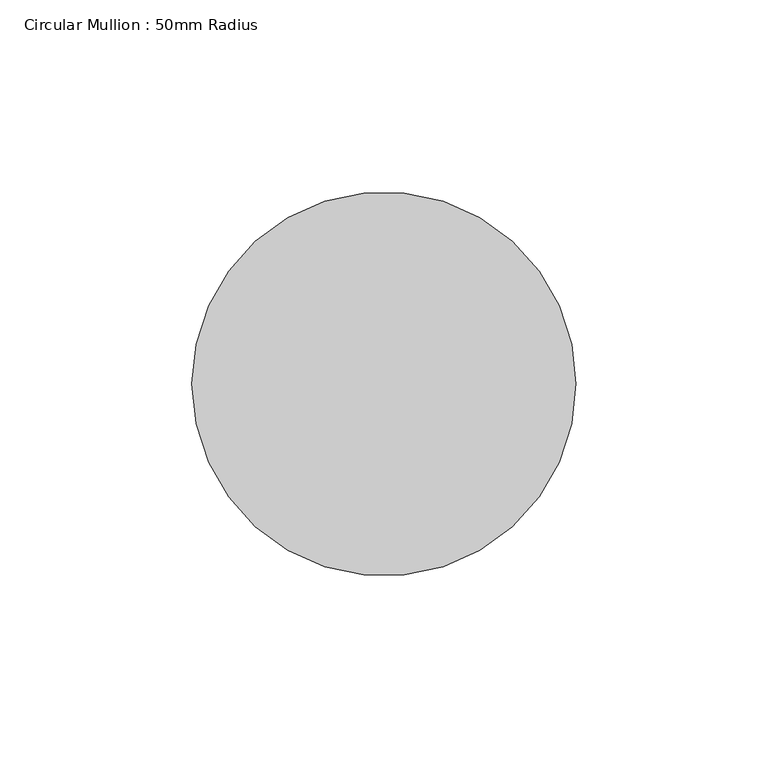
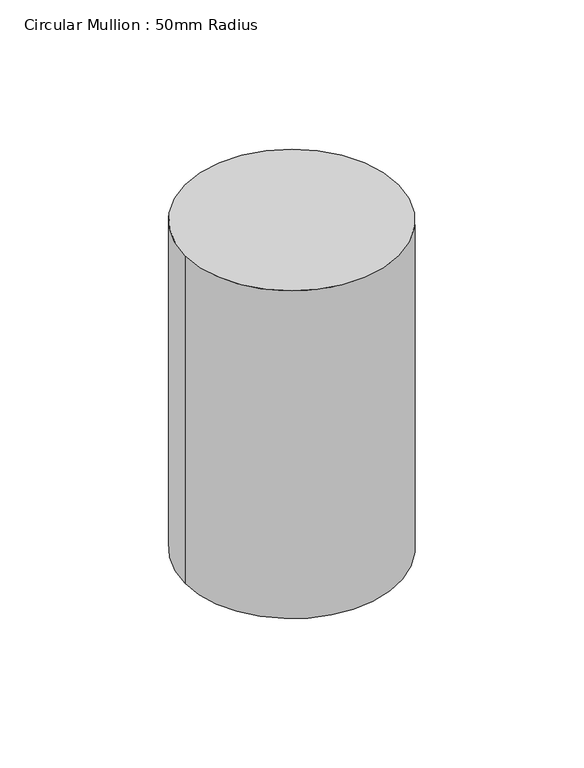
"""IFC4 building model written with IfcOpenShell, lengths in millimetres: member geometry, Circular Mullion : 50mm Radius."""

import ifcopenshell
import ifcopenshell.guid

model = None  # the IFC model being written
_history = None  # IfcOwnerHistory: only IFC2X3 demands one
_inside = {}  # id of a spatial element -> (the spatial element, [elements in it])
_under = {}  # id of a project, library or spatial element -> (it, [spatial elements below it])
_declared = {}  # id of a project -> (the project, [libraries it declares])
_typed = {}  # id of a type object -> (the type object, [elements of that type])
_made_of = {}  # id of a material, layer set ... -> (it, [elements and type objects made of it])


def new_model(schema):
    """Start an empty IFC model of exactly this schema.

    Asked for "IFC4X3", IfcOpenShell would pick the latest addendum, in which some entities
    have other attributes; the version numbers below select the first issue.
    IFC2X3 requires an IfcOwnerHistory on every rooted entity: one is made here for all.
    """
    global model, _history
    if schema == "IFC4X3":
        model = ifcopenshell.file(schema_version=(4, 3, 0, 0))
    else:
        model = ifcopenshell.file(schema=schema)
    _inside.clear()
    _under.clear()
    _declared.clear()
    _typed.clear()
    _made_of.clear()
    _history = None
    if model.schema == "IFC2X3":
        org = make("IfcOrganization", Name="unknown")
        user = make(
            "IfcPersonAndOrganization",
            ThePerson=make("IfcPerson", FamilyName="unknown"),
            TheOrganization=org,
        )
        app = make(
            "IfcApplication",
            ApplicationDeveloper=org,
            Version="unknown",
            ApplicationFullName="unknown",
            ApplicationIdentifier="unknown",
        )
        _history = make(
            "IfcOwnerHistory",
            OwningUser=user,
            OwningApplication=app,
            ChangeAction="ADDED",
            CreationDate=0,
        )
    return model


def make(cls, **values):
    """One entity of the class cls with the attributes given. An attribute that is None is left unset."""
    return model.create_entity(
        cls, **{name: value for name, value in values.items() if value is not None}
    )


def rooted(cls, **values):
    """An entity with a GlobalId (a new one), such as an element, a storey or a relation."""
    return make(cls, GlobalId=ifcopenshell.guid.new(), OwnerHistory=_history, **values)


def si_unit(unit_type, name, prefix=None):
    """IfcSIUnit, for example si_unit("LENGTHUNIT", "METRE", prefix="MILLI")."""
    return make("IfcSIUnit", UnitType=unit_type, Prefix=prefix, Name=name)


def assignment(units):
    """IfcUnitAssignment: the units of a project."""
    return None if units is None else make("IfcUnitAssignment", Units=units)


def point(xyz):
    """IfcCartesianPoint."""
    return None if xyz is None else make("IfcCartesianPoint", Coordinates=xyz)


def direction(xyz):
    """IfcDirection."""
    return None if xyz is None else make("IfcDirection", DirectionRatios=xyz)


def frame(location, z_axis=None, x_axis=None):
    """IfcAxis2Placement3D, a coordinate frame: its origin and axes. An axis left out is left unset."""
    return make(
        "IfcAxis2Placement3D",
        Location=point(location),
        Axis=direction(z_axis),
        RefDirection=direction(x_axis),
    )


def frame_2d(location, x_axis=None):
    """IfcAxis2Placement2D, a coordinate frame in the plane: its origin and x axis."""
    return make(
        "IfcAxis2Placement2D", Location=point(location), RefDirection=direction(x_axis)
    )


def origin():
    """The frame at (0, 0, 0) with its axes left unset."""
    return frame((0.0, 0.0, 0.0))


def origin_2d():
    """The frame at (0, 0) in the plane with its x axis left unset."""
    return frame_2d((0.0, 0.0))


def place(relative_to, where):
    """IfcLocalPlacement: puts the frame where relative to a parent placement (None: the world)."""
    return make(
        "IfcLocalPlacement", PlacementRelTo=relative_to, RelativePlacement=where
    )


def context(
    kind, dimensions, precision=None, world=None, true_north=None, identifier=None
):
    """IfcGeometricRepresentationContext, for example the 3D "Model" context."""
    return make(
        "IfcGeometricRepresentationContext",
        ContextIdentifier=identifier,
        ContextType=kind,
        CoordinateSpaceDimension=dimensions,
        Precision=precision,
        WorldCoordinateSystem=world,
        TrueNorth=true_north,
    )


def project(units=None, contexts=None):
    """IfcProject with its units and contexts."""
    return rooted(
        "IfcProject",
        Name="project",
        RepresentationContexts=contexts,
        UnitsInContext=assignment(units),
    )


def spatial(cls, under=None, at=None, **own):
    """A site, building, storey or space (cls), placed at a placement, below another one or the project."""
    s = rooted(cls, ObjectPlacement=at, **own)
    if under is not None:
        _under.setdefault(under.id(), (under, []))[1].append(s)
    return s


def circle_curve(where, radius):
    """IfcCircle in the frame where."""
    return make("IfcCircle", Position=where, Radius=radius)


def trimmed(basis, trim1, trim2, sense, master):
    """IfcTrimmedCurve: the piece of a basis curve between two trims."""
    return make(
        "IfcTrimmedCurve",
        BasisCurve=basis,
        Trim1=trim1,
        Trim2=trim2,
        SenseAgreement=sense,
        MasterRepresentation=master,
    )


def segment(curve, same_sense, transition):
    """IfcCompositeCurveSegment."""
    return make(
        "IfcCompositeCurveSegment",
        Transition=transition,
        SameSense=same_sense,
        ParentCurve=curve,
    )


def composite_curve(segments, self_intersect=None):
    """IfcCompositeCurve: segments joined end to end."""
    return make("IfcCompositeCurve", Segments=segments, SelfIntersect=self_intersect)


def outline(outer, holes=None, kind="AREA"):
    """IfcArbitraryClosedProfileDef: a profile drawn as a closed curve; with holes, ...WithVoids."""
    if holes is None:
        return make("IfcArbitraryClosedProfileDef", ProfileType=kind, OuterCurve=outer)
    return make(
        "IfcArbitraryProfileDefWithVoids",
        ProfileType=kind,
        OuterCurve=outer,
        InnerCurves=holes,
    )


def extrude(swept, where, along, depth):
    """IfcExtrudedAreaSolid: the profile swept, set in the frame where, extruded along a direction by depth."""
    return make(
        "IfcExtrudedAreaSolid",
        SweptArea=swept,
        Position=where,
        ExtrudedDirection=direction(along),
        Depth=depth,
    )


def shape(context_of_items, identifier, shape_type, items):
    """IfcShapeRepresentation: the items that make up one representation, for example the "Body"."""
    return make(
        "IfcShapeRepresentation",
        ContextOfItems=context_of_items,
        RepresentationIdentifier=identifier,
        RepresentationType=shape_type,
        Items=items,
    )


def source(mapping_origin, context_of_items, identifier, shape_type, items):
    """IfcRepresentationMap: a shape defined once, which mapped items show again and again."""
    return make(
        "IfcRepresentationMap",
        MappingOrigin=mapping_origin,
        MappedRepresentation=shape(context_of_items, identifier, shape_type, items),
    )


def transform(
    local_origin,
    x_axis=None,
    y_axis=None,
    z_axis=None,
    scale=None,
    scale2=None,
    scale3=None,
    uniform=True,
):
    """IfcCartesianTransformationOperator3D, or its non-uniform kind. x_axis, y_axis, z_axis: its Axis1, 2, 3."""
    if uniform:
        return make(
            "IfcCartesianTransformationOperator3D",
            Axis1=direction(x_axis),
            Axis2=direction(y_axis),
            LocalOrigin=point(local_origin),
            Scale=scale,
            Axis3=direction(z_axis),
        )
    return make(
        "IfcCartesianTransformationOperator3DnonUniform",
        Axis1=direction(x_axis),
        Axis2=direction(y_axis),
        LocalOrigin=point(local_origin),
        Scale=scale,
        Axis3=direction(z_axis),
        Scale2=scale2,
        Scale3=scale3,
    )


def mapped(mapping_source, mapping_target):
    """IfcMappedItem: shows the shape of a source again, moved by a transform."""
    return make(
        "IfcMappedItem", MappingSource=mapping_source, MappingTarget=mapping_target
    )


def made_of(thing, what):
    """Note that an element or type object is made of a material, layer set ...; save() writes the relation."""
    if what is not None:
        _made_of.setdefault(what.id(), (what, []))[1].append(thing)
    return thing


def element(
    cls,
    number,
    at=None,
    inside=None,
    cuts=None,
    type_object=None,
    material=None,
    context=None,
    identifier="Body",
    shape_type=None,
    held_by="IfcProductDefinitionShape",
    body=None,
    shapes=None,
    **own,
):
    """One element of the class cls, such as IfcWall. Its Tag is "e" and its number.

    at: its placement. inside: the storey or other place that contains it. cuts: it is an
    opening in that element (IfcRelVoidsElement). A single representation is given by context,
    identifier, shape_type and body (its items); several are given by shapes. held_by: the class
    of the entity that holds the representations. save() writes the other relations.
    """
    e = rooted(cls, Tag="e%d" % number, ObjectPlacement=at, **own)
    if body is not None:
        shapes = [shape(context, identifier, shape_type, body)]
    if shapes is not None:
        e.Representation = make(held_by, Representations=shapes)
    if inside is not None:
        _inside.setdefault(inside.id(), (inside, []))[1].append(e)
    if cuts is not None:
        rooted(
            "IfcRelVoidsElement", RelatingBuildingElement=cuts, RelatedOpeningElement=e
        )
    if type_object is not None:
        _typed.setdefault(type_object.id(), (type_object, []))[1].append(e)
    return made_of(e, material)


def aggregate(whole, parts):
    """IfcRelAggregates: a whole, such as a stair, and the parts it consists of."""
    return rooted("IfcRelAggregates", RelatingObject=whole, RelatedObjects=parts)


def save(model, path):
    """Write the relations noted so far, then the file.

    IfcRelAggregates (storeys below a building ...), IfcRelContainedInSpatialStructure (elements
    in a storey), IfcRelDefinesByType, IfcRelAssociatesMaterial and IfcRelDeclares: one each for
    every whole, place, type object, material and project.
    """
    for whole, parts in _under.values():
        aggregate(whole, parts)
    for where, things in _inside.values():
        rooted(
            "IfcRelContainedInSpatialStructure",
            RelatedElements=things,
            RelatingStructure=where,
        )
    for kind, things in _typed.values():
        rooted("IfcRelDefinesByType", RelatedObjects=things, RelatingType=kind)
    for what, things in _made_of.values():
        rooted("IfcRelAssociatesMaterial", RelatedObjects=things, RelatingMaterial=what)
    for by, libraries in _declared.values():
        rooted("IfcRelDeclares", RelatingContext=by, RelatedDefinitions=libraries)
    model.write(path)


def circular_mullion_50mm_radius_c388bb40(model_context):
    return source(origin(), model_context, "Body", "SweptSolid", [
        extrude(outline(composite_curve([segment(trimmed(circle_curve(origin_2d(), 50.0), [point((50.0, 0.0))], [point((-50.0, 0.0))], False, "CARTESIAN"), True, "CONTINUOUS"), segment(trimmed(circle_curve(origin_2d(), 50.0), [point((-50.0, 0.0))], [point((50.0, 0.0))], False, "CARTESIAN"), True, "CONTINUOUS")], self_intersect=False)), frame((0.0, 0.0, -162.0031267), z_axis=(0.0, 0.0, 1.0), x_axis=(1.0, 0.0, 0.0)), (0.0, 0.0, 1.0), 162.0031267),
    ])


if __name__ == "__main__":
    model = new_model("IFC4")
    model_context = context("Model", 3, world=origin())
    ifc_project = project(units=[si_unit("LENGTHUNIT", "METRE", prefix="MILLI")], contexts=[model_context])
    site = spatial("IfcSite", under=ifc_project)
    building = spatial("IfcBuilding", under=site)
    placement = place(None, origin())
    circular_mullion_50mm_radius_shape = circular_mullion_50mm_radius_c388bb40(model_context)
    element("IfcMember", 1, ObjectType="Circular Mullion : 50mm Radius", at=placement, inside=building, context=model_context, shape_type="MappedRepresentation", body=[
        mapped(circular_mullion_50mm_radius_shape, transform((0.0, 0.0, 0.0), x_axis=(1.0, 0.0, 0.0), y_axis=(0.0, 1.0, 0.0), z_axis=(0.0, 0.0, 1.0))),
    ])
    save(model, "model.ifc")

# Revit data of these elements
# Type "Circular Mullion : 50mm Radius"
#   built-in parameter 1007350 = 0.164042 (stored number, unit not read)
# Element 1 (IfcMember, "Circular Mullion : 50mm Radius")
#   Materials on its faces: "Aluminium"
# Materials
#   "Aluminium": class "Metal", colour RGB 247 247 247, transparency 0, Description = "Aluminium 6061", Cost = 0
